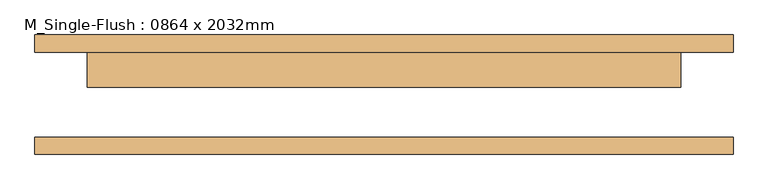
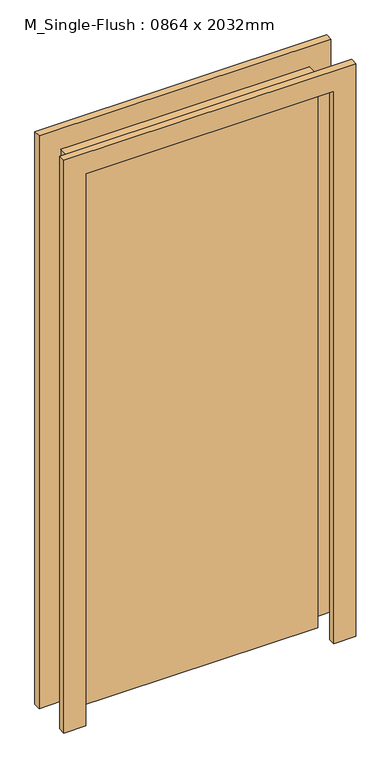
"""IFC4 building model written with IfcOpenShell, lengths in millimetres: door geometry, M_Single-Flush : 0864 x 2032mm."""

from ifc_helpers import new_model, si_unit, frame, origin, origin_with_axes, place, context, project, spatial, polyline, outline, extrude, source, transform, mapped, element, save


def m_single_flush_0864_x_2032mm_f1a57c69(model_context):
    return source(origin(), model_context, "Body", "SweptSolid", [
        extrude(outline(polyline([(2108.0, -508.0), (0.0, -508.0), (0.0, -432.0), (2032.0, -432.0), (2032.0, 432.0), (0.0, 432.0), (0.0, 508.0), (2108.0, 508.0), (2108.0, -508.0)])), frame((0.0, 62.0, 0.0), z_axis=(0.0, 1.0, 0.0), x_axis=(0.0, 0.0, 1.0)), (0.0, 0.0, 1.0), 25.0),
        extrude(outline(polyline([(2108.0, 508.0), (2108.0, -508.0), (0.0, -508.0), (0.0, -432.0), (2032.0, -432.0), (2032.0, 432.0), (0.0, 432.0), (0.0, 508.0), (2108.0, 508.0)])), frame((0.0, -87.0, 0.0), z_axis=(0.0, 1.0, 0.0), x_axis=(0.0, 0.0, 1.0)), (0.0, 0.0, 1.0), 25.0),
        extrude(outline(polyline([(432.0, 11.0), (-432.0, 11.0), (-432.0, 62.0), (432.0, 62.0), (432.0, 11.0)])), origin_with_axes(), (0.0, 0.0, 1.0), 2032.0),
    ])


if __name__ == "__main__":
    model = new_model("IFC4")
    model_context = context("Model", 3, world=origin())
    ifc_project = project(units=[si_unit("LENGTHUNIT", "METRE", prefix="MILLI")], contexts=[model_context])
    site = spatial("IfcSite", under=ifc_project)
    building = spatial("IfcBuilding", under=site)
    placement = place(None, origin())
    m_single_flush_0864_x_2032mm_shape = m_single_flush_0864_x_2032mm_f1a57c69(model_context)
    element("IfcDoor", 1, ObjectType="M_Single-Flush : 0864 x 2032mm", at=placement, inside=building, context=model_context, shape_type="MappedRepresentation", body=[
        mapped(m_single_flush_0864_x_2032mm_shape, transform((0.0, 0.0, 0.0), x_axis=(1.0, 0.0, 0.0), y_axis=(0.0, 1.0, 0.0), z_axis=(0.0, 0.0, 1.0))),
    ])
    save(model, "model.ifc")

# Revit data of these elements
# Type "M_Single-Flush : 0864 x 2032mm"
#   Manufacturer = "Manufacturer"
#   Type Mark = "32"
#   Construction Type = "Construction Type"
#   Fire Rating = "Fire Rating"
#   AccessibilityPerformance = "AccessibilityPerformance"
#   CodePerformance = "CodePerformance"
#   IsFireExit = "IsFireExit"
#   ConstructionType = "ConstructionType"
#   GlazingAreaFraction = "GlazingAreaFraction"
#   OperationType = "OperationType"
#   Area = "Area"
#   Color = "Color"
#   Constituents = "Constituents"
#   Features = "Features"
#   Finish = "Finish"
#   Grade = "Grade"
#   Material = "Material"
#   ModelReference = "ModelReference"
#   NominalHeight = "NominalHeight"
#   NominalLength = "NominalLength"
#   NominalWidth = "NominalWidth"
#   ProductionYear = "ProductionYear"
#   Reference = "Reference"
#   Shape = "Shape"
#   Size = "Size"
#   SustainabilityPerformance = "SustainabilityPerformance"
#   WarrantyDescription = "WarrantyDescription"
#   WarrantyDurationLabor = "WarrantyDurationLabor"
#   WarrantyDurationParts = "WarrantyDurationParts"
#   WarrantyGuarantorLabor = "WarrantyGuarantorLabor"
#   WarrantyGuarantorParts = "WarrantyGuarantorParts"
#   ExpectedLife = "ExpectedLife"
#   ReplacementCost = "ReplacementCost"
#   AssetAccountingType = "FIXED"
#   ModelLabel = "ModelLabel"
#   Thickness = 0.051 m
#   Height = 2.032 m
#   Trim Projection Ext = 0.025 m
#   Trim Projection Int = 0.025 m
#   Trim Width = 0.076 m
#   Width = 0.864 m
#   Door Material = Door - Panel
#   Frame Material = Door - Frame
#   Function = (empty or 0)
#   Wall Closure = (empty or 0)
# Element 1 (IfcDoor, "M_Single-Flush : 0864 x 2032mm")
#   Materials on its faces: "Door - Frame", "Door - Panel"
# Materials
#   "Door - Panel": class "Wood", colour RGB 210 159 95, transparency 0
#   "Door - Frame": class "Miscellaneous", colour RGB 118 70 51, transparency 0
